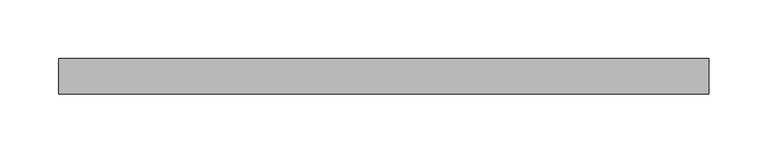
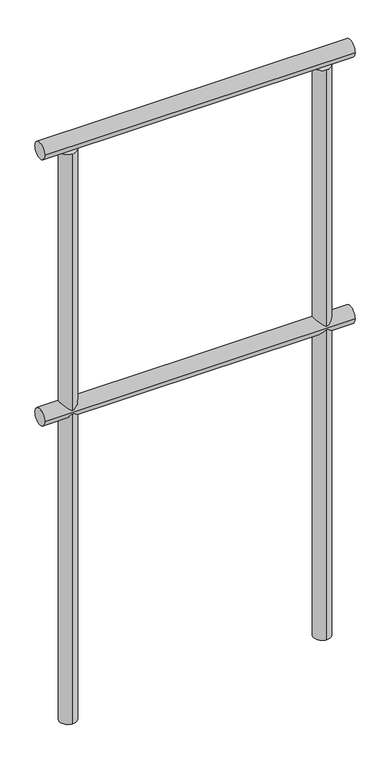
"""IFC4 building model written with IfcOpenShell, lengths in millimetres: railing geometry."""

from ifc_helpers import new_model, si_unit, point, frame, frame_2d, origin, place, context, project, spatial, circle_curve, trimmed, segment, composite_curve, outline, extrude, source, transform, mapped, element, save


def railing_c9c19dc0(model_context):
    return source(origin(), model_context, "Body", "SweptSolid", [
        extrude(outline(composite_curve([segment(trimmed(circle_curve(frame_2d((48139.2482382, 885.0)), 15.0), [point((48124.2482382, 885.0))], [point((48154.2482382, 885.0))], False, "CARTESIAN"), True, "CONTINUOUS"), segment(trimmed(circle_curve(frame_2d((48139.2482382, 885.0)), 15.0), [point((48154.2482382, 885.0))], [point((48124.2482382, 885.0))], False, "CARTESIAN"), True, "CONTINUOUS")], self_intersect=False)), frame((-1001.4, 0.0, 0.0), z_axis=(1.0, 0.0, 0.0), x_axis=(0.0, 1.0, 0.0)), (0.0, 0.0, 1.0), 551.4),
        extrude(outline(composite_curve([segment(trimmed(circle_curve(frame_2d((48139.2482382, 1385.0)), 15.0), [point((48124.2482382, 1385.0))], [point((48154.2482382, 1385.0))], False, "CARTESIAN"), True, "CONTINUOUS"), segment(trimmed(circle_curve(frame_2d((48139.2482382, 1385.0)), 15.0), [point((48154.2482382, 1385.0))], [point((48124.2482382, 1385.0))], False, "CARTESIAN"), True, "CONTINUOUS")], self_intersect=False)), frame((-1001.4, 0.0, 0.0), z_axis=(1.0, 0.0, 0.0), x_axis=(0.0, 1.0, 0.0)), (0.0, 0.0, 1.0), 551.4),
        extrude(outline(composite_curve([segment(trimmed(circle_curve(frame_2d((-500.0, 48139.2482382)), 15.0), [point((-500.0, 48124.2482382))], [point((-500.0, 48154.2482382))], False, "CARTESIAN"), True, "CONTINUOUS"), segment(trimmed(circle_curve(frame_2d((-500.0, 48139.2482382)), 15.0), [point((-500.0, 48154.2482382))], [point((-500.0, 48124.2482382))], False, "CARTESIAN"), True, "CONTINUOUS")], self_intersect=False)), frame((0.0, 0.0, 300.0), z_axis=(0.0, 0.0, 1.0), x_axis=(1.0, 0.0, 0.0)), (0.0, 0.0, 1.0), 1070.0),
        extrude(outline(composite_curve([segment(trimmed(circle_curve(frame_2d((-951.4, 48139.2482382)), 15.0), [point((-951.4, 48124.2482382))], [point((-951.4, 48154.2482382))], False, "CARTESIAN"), True, "CONTINUOUS"), segment(trimmed(circle_curve(frame_2d((-951.4, 48139.2482382)), 15.0), [point((-951.4, 48154.2482382))], [point((-951.4, 48124.2482382))], False, "CARTESIAN"), True, "CONTINUOUS")], self_intersect=False)), frame((0.0, 0.0, 300.0), z_axis=(0.0, 0.0, 1.0), x_axis=(1.0, 0.0, 0.0)), (0.0, 0.0, 1.0), 1070.0),
    ])


if __name__ == "__main__":
    model = new_model("IFC4")
    model_context = context("Model", 3, world=origin())
    ifc_project = project(units=[si_unit("LENGTHUNIT", "METRE", prefix="MILLI")], contexts=[model_context])
    site = spatial("IfcSite", under=ifc_project)
    building = spatial("IfcBuilding", under=site)
    placement = place(None, origin())
    railing_shape = railing_c9c19dc0(model_context)
    element("IfcRailing", 1, at=placement, inside=building, context=model_context, shape_type="MappedRepresentation", body=[
        mapped(railing_shape, transform((0.0, 0.0, 0.0), x_axis=(1.0, 0.0, 0.0), y_axis=(0.0, 1.0, 0.0), z_axis=(0.0, 0.0, 1.0))),
    ])
    save(model, "model.ifc")
